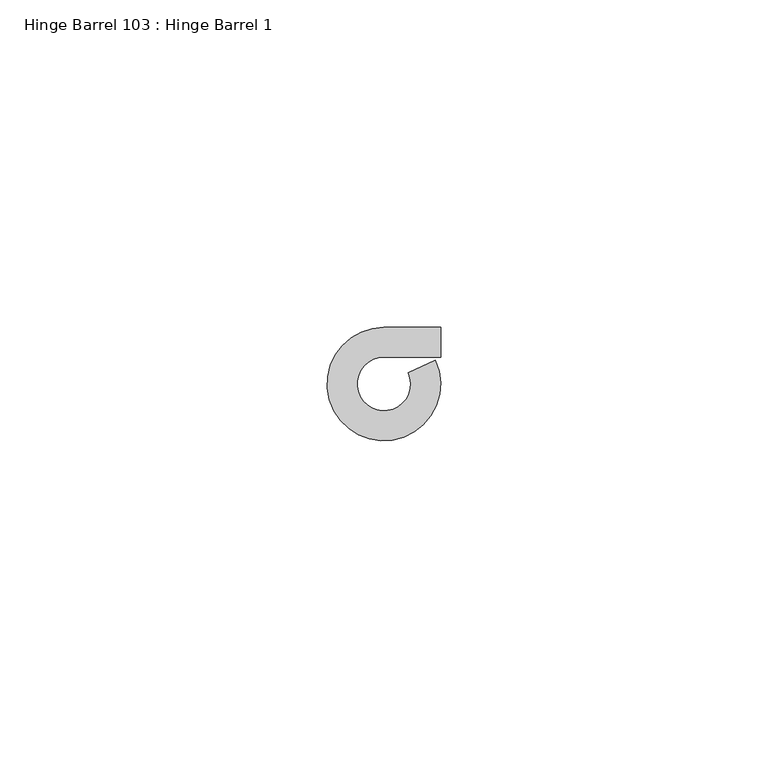
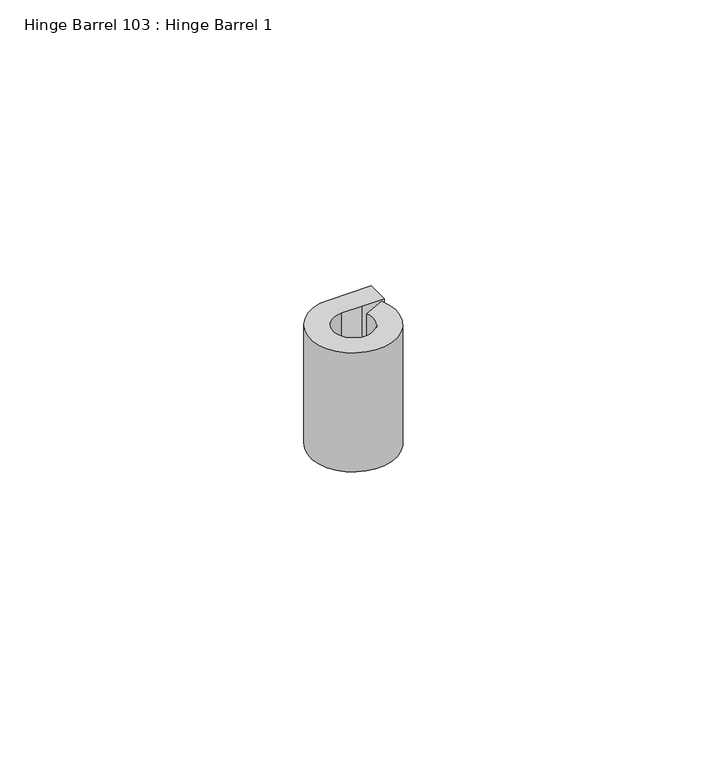
"""IFC4 building model written with IfcOpenShell, lengths in millimetres: proxy geometry, Hinge Barrel 103 : Hinge Barrel 1."""

from ifc_helpers import new_model, si_unit, point, frame, frame_2d, origin, place, context, project, spatial, polyline, circle_curve, trimmed, segment, composite_curve, outline, extrude, source, transform, mapped, element, save


def hinge_barrel_103_hinge_barrel_1_f2478639(model_context):
    return source(origin(), model_context, "Body", "SweptSolid", [
        extrude(outline(composite_curve([segment(polyline([(587323.2214739, -533980.5883841), (587319.1320739, -533980.5883841)]), True, "CONTINUOUS"), segment(trimmed(circle_curve(frame_2d((587319.1320739, -533984.6777841)), 4.0894), [point((587319.1320739, -533980.5883841))], [point((587322.8436736, -533982.9610371))], True, "CARTESIAN"), True, "CONTINUOUS"), segment(polyline([(587322.8436736, -533982.9610371), (587326.986084, -533981.0450249)]), True, "CONTINUOUS"), segment(trimmed(circle_curve(frame_2d((587319.1320739, -533984.6777841)), 8.6534625), [point((587326.986084, -533981.0450249))], [point((587319.1320739, -533976.0243216))], False, "CARTESIAN"), True, "CONTINUOUS"), segment(polyline([(587319.1320739, -533976.0243216), (587327.7934739, -533976.0243216), (587327.7934739, -533980.5883841), (587323.2214739, -533980.5883841)]), True, "CONTINUOUS")], self_intersect=False)), frame((0.0, 0.0, 1123.95), z_axis=(0.0, 0.0, 1.0), x_axis=(1.0, 0.0, 0.0)), (0.0, 0.0, 1.0), 25.4),
    ])


if __name__ == "__main__":
    model = new_model("IFC4")
    model_context = context("Model", 3, world=origin())
    ifc_project = project(units=[si_unit("LENGTHUNIT", "METRE", prefix="MILLI")], contexts=[model_context])
    site = spatial("IfcSite", under=ifc_project)
    building = spatial("IfcBuilding", under=site)
    placement = place(None, origin())
    hinge_barrel_103_hinge_barrel_1_shape = hinge_barrel_103_hinge_barrel_1_f2478639(model_context)
    element("IfcBuildingElementProxy", 1, Name="Hinge Barrel 103 : Hinge Barrel 1", ObjectType="Hinge Barrel 103 : Hinge Barrel 1", at=placement, inside=building, context=model_context, shape_type="MappedRepresentation", body=[
        mapped(hinge_barrel_103_hinge_barrel_1_shape, transform((0.0, 0.0, 0.0), x_axis=(1.0, 0.0, 0.0), y_axis=(0.0, 1.0, 0.0), z_axis=(0.0, 0.0, 1.0))),
    ])
    save(model, "model.ifc")

# Revit data of these elements
# Element 1 (IfcBuildingElementProxy, "Hinge Barrel 103 : Hinge Barrel 1")
#   Materials on its faces: "6\"X6\" WELD-ON STL BUTT HINGE"
# Materials
#   "6\"X6\" WELD-ON STL BUTT HINGE": class "Metal", colour RGB 189 187 185, transparency 0, Description = "Carbon steel", Cost = 0
